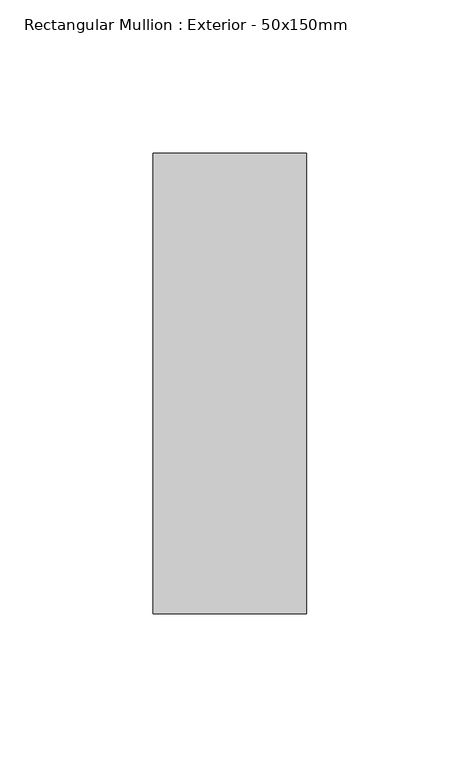
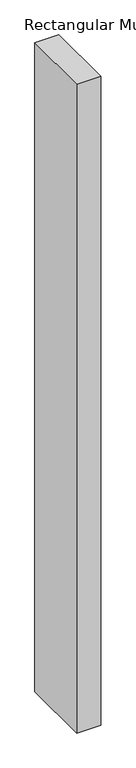
"""IFC4 building model written with IfcOpenShell, lengths in millimetres: member geometry, Rectangular Mullion : Exterior - 50x150mm."""

import ifcopenshell
import ifcopenshell.guid

model = None  # the IFC model being written
_history = None  # IfcOwnerHistory: only IFC2X3 demands one
_inside = {}  # id of a spatial element -> (the spatial element, [elements in it])
_under = {}  # id of a project, library or spatial element -> (it, [spatial elements below it])
_declared = {}  # id of a project -> (the project, [libraries it declares])
_typed = {}  # id of a type object -> (the type object, [elements of that type])
_made_of = {}  # id of a material, layer set ... -> (it, [elements and type objects made of it])


def new_model(schema):
    """Start an empty IFC model of exactly this schema.

    Asked for "IFC4X3", IfcOpenShell would pick the latest addendum, in which some entities
    have other attributes; the version numbers below select the first issue.
    IFC2X3 requires an IfcOwnerHistory on every rooted entity: one is made here for all.
    """
    global model, _history
    if schema == "IFC4X3":
        model = ifcopenshell.file(schema_version=(4, 3, 0, 0))
    else:
        model = ifcopenshell.file(schema=schema)
    _inside.clear()
    _under.clear()
    _declared.clear()
    _typed.clear()
    _made_of.clear()
    _history = None
    if model.schema == "IFC2X3":
        org = make("IfcOrganization", Name="unknown")
        user = make(
            "IfcPersonAndOrganization",
            ThePerson=make("IfcPerson", FamilyName="unknown"),
            TheOrganization=org,
        )
        app = make(
            "IfcApplication",
            ApplicationDeveloper=org,
            Version="unknown",
            ApplicationFullName="unknown",
            ApplicationIdentifier="unknown",
        )
        _history = make(
            "IfcOwnerHistory",
            OwningUser=user,
            OwningApplication=app,
            ChangeAction="ADDED",
            CreationDate=0,
        )
    return model


def make(cls, **values):
    """One entity of the class cls with the attributes given. An attribute that is None is left unset."""
    return model.create_entity(
        cls, **{name: value for name, value in values.items() if value is not None}
    )


def rooted(cls, **values):
    """An entity with a GlobalId (a new one), such as an element, a storey or a relation."""
    return make(cls, GlobalId=ifcopenshell.guid.new(), OwnerHistory=_history, **values)


def si_unit(unit_type, name, prefix=None):
    """IfcSIUnit, for example si_unit("LENGTHUNIT", "METRE", prefix="MILLI")."""
    return make("IfcSIUnit", UnitType=unit_type, Prefix=prefix, Name=name)


def assignment(units):
    """IfcUnitAssignment: the units of a project."""
    return None if units is None else make("IfcUnitAssignment", Units=units)


def point(xyz):
    """IfcCartesianPoint."""
    return None if xyz is None else make("IfcCartesianPoint", Coordinates=xyz)


def direction(xyz):
    """IfcDirection."""
    return None if xyz is None else make("IfcDirection", DirectionRatios=xyz)


def frame(location, z_axis=None, x_axis=None):
    """IfcAxis2Placement3D, a coordinate frame: its origin and axes. An axis left out is left unset."""
    return make(
        "IfcAxis2Placement3D",
        Location=point(location),
        Axis=direction(z_axis),
        RefDirection=direction(x_axis),
    )


def origin():
    """The frame at (0, 0, 0) with its axes left unset."""
    return frame((0.0, 0.0, 0.0))


def place(relative_to, where):
    """IfcLocalPlacement: puts the frame where relative to a parent placement (None: the world)."""
    return make(
        "IfcLocalPlacement", PlacementRelTo=relative_to, RelativePlacement=where
    )


def context(
    kind, dimensions, precision=None, world=None, true_north=None, identifier=None
):
    """IfcGeometricRepresentationContext, for example the 3D "Model" context."""
    return make(
        "IfcGeometricRepresentationContext",
        ContextIdentifier=identifier,
        ContextType=kind,
        CoordinateSpaceDimension=dimensions,
        Precision=precision,
        WorldCoordinateSystem=world,
        TrueNorth=true_north,
    )


def project(units=None, contexts=None):
    """IfcProject with its units and contexts."""
    return rooted(
        "IfcProject",
        Name="project",
        RepresentationContexts=contexts,
        UnitsInContext=assignment(units),
    )


def spatial(cls, under=None, at=None, **own):
    """A site, building, storey or space (cls), placed at a placement, below another one or the project."""
    s = rooted(cls, ObjectPlacement=at, **own)
    if under is not None:
        _under.setdefault(under.id(), (under, []))[1].append(s)
    return s


def polyline(points):
    """IfcPolyline through the points."""
    return make("IfcPolyline", Points=[point(p) for p in points])


def outline(outer, holes=None, kind="AREA"):
    """IfcArbitraryClosedProfileDef: a profile drawn as a closed curve; with holes, ...WithVoids."""
    if holes is None:
        return make("IfcArbitraryClosedProfileDef", ProfileType=kind, OuterCurve=outer)
    return make(
        "IfcArbitraryProfileDefWithVoids",
        ProfileType=kind,
        OuterCurve=outer,
        InnerCurves=holes,
    )


def extrude(swept, where, along, depth):
    """IfcExtrudedAreaSolid: the profile swept, set in the frame where, extruded along a direction by depth."""
    return make(
        "IfcExtrudedAreaSolid",
        SweptArea=swept,
        Position=where,
        ExtrudedDirection=direction(along),
        Depth=depth,
    )


def shape(context_of_items, identifier, shape_type, items):
    """IfcShapeRepresentation: the items that make up one representation, for example the "Body"."""
    return make(
        "IfcShapeRepresentation",
        ContextOfItems=context_of_items,
        RepresentationIdentifier=identifier,
        RepresentationType=shape_type,
        Items=items,
    )


def source(mapping_origin, context_of_items, identifier, shape_type, items):
    """IfcRepresentationMap: a shape defined once, which mapped items show again and again."""
    return make(
        "IfcRepresentationMap",
        MappingOrigin=mapping_origin,
        MappedRepresentation=shape(context_of_items, identifier, shape_type, items),
    )


def transform(
    local_origin,
    x_axis=None,
    y_axis=None,
    z_axis=None,
    scale=None,
    scale2=None,
    scale3=None,
    uniform=True,
):
    """IfcCartesianTransformationOperator3D, or its non-uniform kind. x_axis, y_axis, z_axis: its Axis1, 2, 3."""
    if uniform:
        return make(
            "IfcCartesianTransformationOperator3D",
            Axis1=direction(x_axis),
            Axis2=direction(y_axis),
            LocalOrigin=point(local_origin),
            Scale=scale,
            Axis3=direction(z_axis),
        )
    return make(
        "IfcCartesianTransformationOperator3DnonUniform",
        Axis1=direction(x_axis),
        Axis2=direction(y_axis),
        LocalOrigin=point(local_origin),
        Scale=scale,
        Axis3=direction(z_axis),
        Scale2=scale2,
        Scale3=scale3,
    )


def mapped(mapping_source, mapping_target):
    """IfcMappedItem: shows the shape of a source again, moved by a transform."""
    return make(
        "IfcMappedItem", MappingSource=mapping_source, MappingTarget=mapping_target
    )


def made_of(thing, what):
    """Note that an element or type object is made of a material, layer set ...; save() writes the relation."""
    if what is not None:
        _made_of.setdefault(what.id(), (what, []))[1].append(thing)
    return thing


def element(
    cls,
    number,
    at=None,
    inside=None,
    cuts=None,
    type_object=None,
    material=None,
    context=None,
    identifier="Body",
    shape_type=None,
    held_by="IfcProductDefinitionShape",
    body=None,
    shapes=None,
    **own,
):
    """One element of the class cls, such as IfcWall. Its Tag is "e" and its number.

    at: its placement. inside: the storey or other place that contains it. cuts: it is an
    opening in that element (IfcRelVoidsElement). A single representation is given by context,
    identifier, shape_type and body (its items); several are given by shapes. held_by: the class
    of the entity that holds the representations. save() writes the other relations.
    """
    e = rooted(cls, Tag="e%d" % number, ObjectPlacement=at, **own)
    if body is not None:
        shapes = [shape(context, identifier, shape_type, body)]
    if shapes is not None:
        e.Representation = make(held_by, Representations=shapes)
    if inside is not None:
        _inside.setdefault(inside.id(), (inside, []))[1].append(e)
    if cuts is not None:
        rooted(
            "IfcRelVoidsElement", RelatingBuildingElement=cuts, RelatedOpeningElement=e
        )
    if type_object is not None:
        _typed.setdefault(type_object.id(), (type_object, []))[1].append(e)
    return made_of(e, material)


def aggregate(whole, parts):
    """IfcRelAggregates: a whole, such as a stair, and the parts it consists of."""
    return rooted("IfcRelAggregates", RelatingObject=whole, RelatedObjects=parts)


def save(model, path):
    """Write the relations noted so far, then the file.

    IfcRelAggregates (storeys below a building ...), IfcRelContainedInSpatialStructure (elements
    in a storey), IfcRelDefinesByType, IfcRelAssociatesMaterial and IfcRelDeclares: one each for
    every whole, place, type object, material and project.
    """
    for whole, parts in _under.values():
        aggregate(whole, parts)
    for where, things in _inside.values():
        rooted(
            "IfcRelContainedInSpatialStructure",
            RelatedElements=things,
            RelatingStructure=where,
        )
    for kind, things in _typed.values():
        rooted("IfcRelDefinesByType", RelatedObjects=things, RelatingType=kind)
    for what, things in _made_of.values():
        rooted("IfcRelAssociatesMaterial", RelatedObjects=things, RelatingMaterial=what)
    for by, libraries in _declared.values():
        rooted("IfcRelDeclares", RelatingContext=by, RelatedDefinitions=libraries)
    model.write(path)


def rectangular_mullion_exterior_50x150mm_ae104826(model_context):
    return source(origin(), model_context, "Body", "SweptSolid", [
        extrude(outline(polyline([(25.0, 0.0), (25.0, -150.0), (-25.0, -150.0), (-25.0, 0.0), (25.0, 0.0)])), frame((0.0, 0.0, -1425.0000002), z_axis=(0.0, 0.0, 1.0), x_axis=(1.0, 0.0, 0.0)), (0.0, 0.0, 1.0), 1425.0000002),
    ])


if __name__ == "__main__":
    model = new_model("IFC4")
    model_context = context("Model", 3, world=origin())
    ifc_project = project(units=[si_unit("LENGTHUNIT", "METRE", prefix="MILLI")], contexts=[model_context])
    site = spatial("IfcSite", under=ifc_project)
    building = spatial("IfcBuilding", under=site)
    placement = place(None, origin())
    rectangular_mullion_exterior_50x150mm_shape = rectangular_mullion_exterior_50x150mm_ae104826(model_context)
    element("IfcMember", 1, ObjectType="Rectangular Mullion : Exterior - 50x150mm", at=placement, inside=building, context=model_context, shape_type="MappedRepresentation", body=[
        mapped(rectangular_mullion_exterior_50x150mm_shape, transform((0.0, 0.0, 0.0), x_axis=(1.0, 0.0, 0.0), y_axis=(0.0, 1.0, 0.0), z_axis=(0.0, 0.0, 1.0))),
    ])
    save(model, "model.ifc")

# Revit data of these elements
# Type "Rectangular Mullion : Exterior - 50x150mm"
#   built-in parameter 1007351 = -0.246063 (stored number, unit not read)
#   built-in parameter 1007304 = 0.492126 (stored number, unit not read)
#   built-in parameter 1007301 = 0.082021 (stored number, unit not read)
#   built-in parameter 1007300 = 0.082021 (stored number, unit not read)
# Element 1 (IfcMember, "Rectangular Mullion : Exterior - 50x150mm")
#   Materials on its faces: "Default Frame/Mullion (Interior/Exterior)"
# Materials
#   "Default Frame/Mullion (Interior/Exterior)": class "Generic", colour RGB 205 205 205, transparency 0, Description = "Udefineret karm/ramme materiale", Cost = 0
